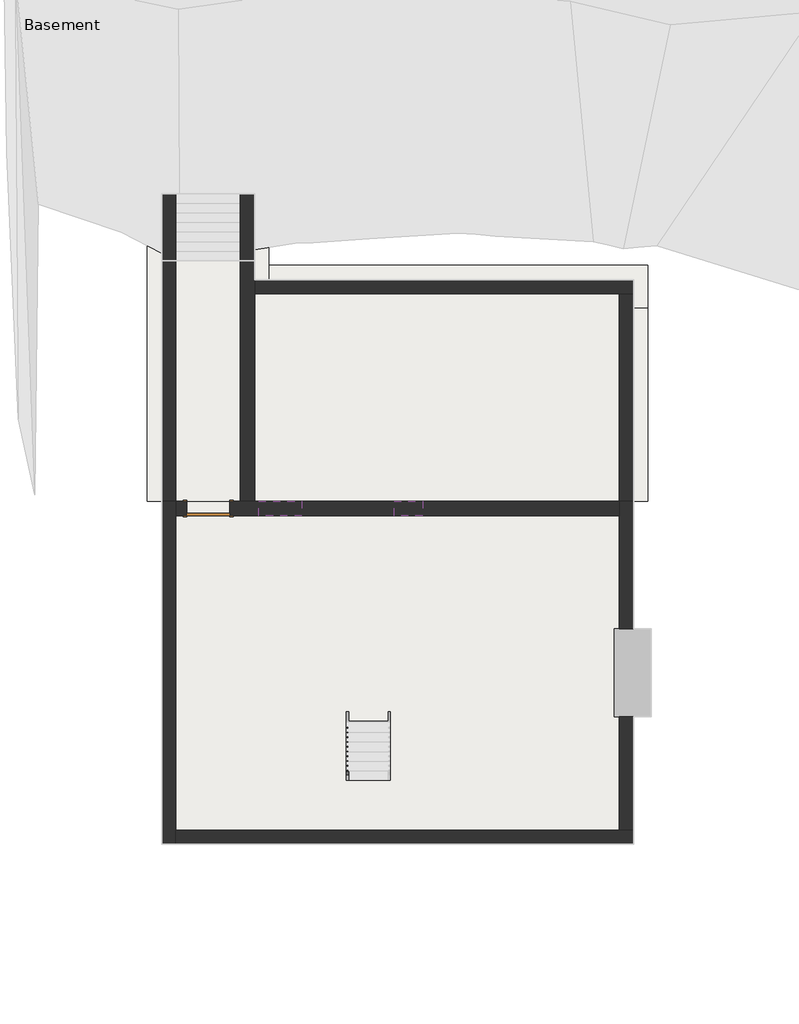
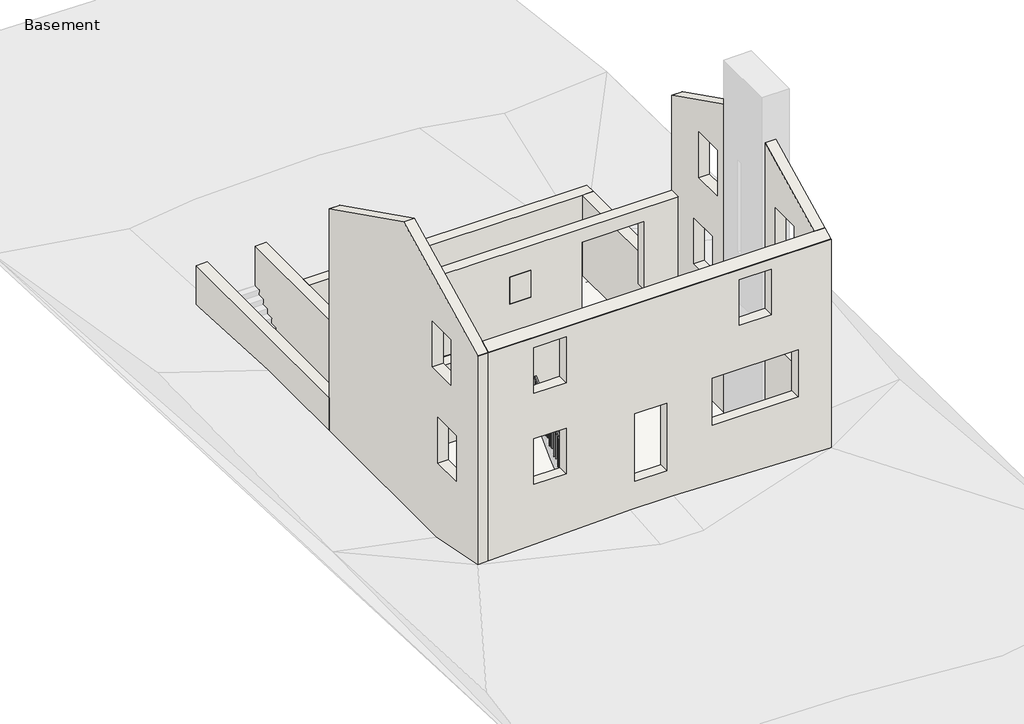
# One storey, part 1 of 2: 11 walls, 4 footings, 4 slabs, 1 door, 1 railing.
"""IFC4 building model written with IfcOpenShell, lengths in millimetres."""

import ifcopenshell
import ifcopenshell.guid

model = None  # the IFC model being written
_history = None  # IfcOwnerHistory: only IFC2X3 demands one
_inside = {}  # id of a spatial element -> (the spatial element, [elements in it])
_under = {}  # id of a project, library or spatial element -> (it, [spatial elements below it])
_declared = {}  # id of a project -> (the project, [libraries it declares])
_typed = {}  # id of a type object -> (the type object, [elements of that type])
_made_of = {}  # id of a material, layer set ... -> (it, [elements and type objects made of it])


def new_model(schema):
    """Start an empty IFC model of exactly this schema.

    Asked for "IFC4X3", IfcOpenShell would pick the latest addendum, in which some entities
    have other attributes; the version numbers below select the first issue.
    IFC2X3 requires an IfcOwnerHistory on every rooted entity: one is made here for all.
    """
    global model, _history
    if schema == "IFC4X3":
        model = ifcopenshell.file(schema_version=(4, 3, 0, 0))
    else:
        model = ifcopenshell.file(schema=schema)
    _inside.clear()
    _under.clear()
    _declared.clear()
    _typed.clear()
    _made_of.clear()
    _history = None
    if model.schema == "IFC2X3":
        org = make("IfcOrganization", Name="unknown")
        user = make(
            "IfcPersonAndOrganization",
            ThePerson=make("IfcPerson", FamilyName="unknown"),
            TheOrganization=org,
        )
        app = make(
            "IfcApplication",
            ApplicationDeveloper=org,
            Version="unknown",
            ApplicationFullName="unknown",
            ApplicationIdentifier="unknown",
        )
        _history = make(
            "IfcOwnerHistory",
            OwningUser=user,
            OwningApplication=app,
            ChangeAction="ADDED",
            CreationDate=0,
        )
    return model


def make(cls, **values):
    """One entity of the class cls with the attributes given. An attribute that is None is left unset."""
    return model.create_entity(
        cls, **{name: value for name, value in values.items() if value is not None}
    )


def rooted(cls, **values):
    """An entity with a GlobalId (a new one), such as an element, a storey or a relation."""
    return make(cls, GlobalId=ifcopenshell.guid.new(), OwnerHistory=_history, **values)


def si_unit(unit_type, name, prefix=None):
    """IfcSIUnit, for example si_unit("LENGTHUNIT", "METRE", prefix="MILLI")."""
    return make("IfcSIUnit", UnitType=unit_type, Prefix=prefix, Name=name)


def assignment(units):
    """IfcUnitAssignment: the units of a project."""
    return None if units is None else make("IfcUnitAssignment", Units=units)


def point(xyz):
    """IfcCartesianPoint."""
    return None if xyz is None else make("IfcCartesianPoint", Coordinates=xyz)


def direction(xyz):
    """IfcDirection."""
    return None if xyz is None else make("IfcDirection", DirectionRatios=xyz)


def frame(location, z_axis=None, x_axis=None):
    """IfcAxis2Placement3D, a coordinate frame: its origin and axes. An axis left out is left unset."""
    return make(
        "IfcAxis2Placement3D",
        Location=point(location),
        Axis=direction(z_axis),
        RefDirection=direction(x_axis),
    )


def origin():
    """The frame at (0, 0, 0) with its axes left unset."""
    return frame((0.0, 0.0, 0.0))


def origin_with_axes():
    """The frame at (0, 0, 0) with the z axis (0, 0, 1) and the x axis (1, 0, 0) written out."""
    return frame((0.0, 0.0, 0.0), z_axis=(0.0, 0.0, 1.0), x_axis=(1.0, 0.0, 0.0))


def place(relative_to, where):
    """IfcLocalPlacement: puts the frame where relative to a parent placement (None: the world)."""
    return make(
        "IfcLocalPlacement", PlacementRelTo=relative_to, RelativePlacement=where
    )


def context(
    kind, dimensions, precision=None, world=None, true_north=None, identifier=None
):
    """IfcGeometricRepresentationContext, for example the 3D "Model" context."""
    return make(
        "IfcGeometricRepresentationContext",
        ContextIdentifier=identifier,
        ContextType=kind,
        CoordinateSpaceDimension=dimensions,
        Precision=precision,
        WorldCoordinateSystem=world,
        TrueNorth=true_north,
    )


def project(units=None, contexts=None):
    """IfcProject with its units and contexts."""
    return rooted(
        "IfcProject",
        Name="project",
        RepresentationContexts=contexts,
        UnitsInContext=assignment(units),
    )


def spatial(cls, under=None, at=None, **own):
    """A site, building, storey or space (cls), placed at a placement, below another one or the project."""
    s = rooted(cls, ObjectPlacement=at, **own)
    if under is not None:
        _under.setdefault(under.id(), (under, []))[1].append(s)
    return s


def polyline(points):
    """IfcPolyline through the points."""
    return make("IfcPolyline", Points=[point(p) for p in points])


def outline(outer, holes=None, kind="AREA"):
    """IfcArbitraryClosedProfileDef: a profile drawn as a closed curve; with holes, ...WithVoids."""
    if holes is None:
        return make("IfcArbitraryClosedProfileDef", ProfileType=kind, OuterCurve=outer)
    return make(
        "IfcArbitraryProfileDefWithVoids",
        ProfileType=kind,
        OuterCurve=outer,
        InnerCurves=holes,
    )


def extrude(swept, where, along, depth):
    """IfcExtrudedAreaSolid: the profile swept, set in the frame where, extruded along a direction by depth."""
    return make(
        "IfcExtrudedAreaSolid",
        SweptArea=swept,
        Position=where,
        ExtrudedDirection=direction(along),
        Depth=depth,
    )


def faces_of(points, faces, orient=None, outer=None):
    """IfcFace entities. A face is a list of loops; a loop is a list of indices into points, from 0.

    orient and outer hold one flag for each loop. By default every Orientation is true, the
    first loop of a face is its IfcFaceOuterBound and the others are IfcFaceBound.
    """
    made = []
    for i, loops in enumerate(faces):
        bounds = []
        for j, loop in enumerate(loops):
            is_outer = j == 0 if outer is None else outer[i][j]
            bounds.append(
                make(
                    "IfcFaceOuterBound" if is_outer else "IfcFaceBound",
                    Bound=make("IfcPolyLoop", Polygon=[points[k] for k in loop]),
                    Orientation=True if orient is None else orient[i][j],
                )
            )
        made.append(make("IfcFace", Bounds=bounds))
    return made


def faceted_brep(points, faces, orient=None, outer=None, voids=None):
    """IfcFacetedBrep: a solid bounded by flat faces; with voids (closed shells), ...WithVoids."""
    shared = [point(p) for p in points]
    hull = make("IfcClosedShell", CfsFaces=faces_of(shared, faces, orient, outer))
    if voids is None:
        return make("IfcFacetedBrep", Outer=hull)
    return make(
        "IfcFacetedBrepWithVoids",
        Outer=hull,
        Voids=[
            make(cls, CfsFaces=faces_of(shared, fs, o, b)) for cls, fs, o, b in voids
        ],
    )


def shape(context_of_items, identifier, shape_type, items):
    """IfcShapeRepresentation: the items that make up one representation, for example the "Body"."""
    return make(
        "IfcShapeRepresentation",
        ContextOfItems=context_of_items,
        RepresentationIdentifier=identifier,
        RepresentationType=shape_type,
        Items=items,
    )


def source(mapping_origin, context_of_items, identifier, shape_type, items):
    """IfcRepresentationMap: a shape defined once, which mapped items show again and again."""
    return make(
        "IfcRepresentationMap",
        MappingOrigin=mapping_origin,
        MappedRepresentation=shape(context_of_items, identifier, shape_type, items),
    )


def transform(
    local_origin,
    x_axis=None,
    y_axis=None,
    z_axis=None,
    scale=None,
    scale2=None,
    scale3=None,
    uniform=True,
):
    """IfcCartesianTransformationOperator3D, or its non-uniform kind. x_axis, y_axis, z_axis: its Axis1, 2, 3."""
    if uniform:
        return make(
            "IfcCartesianTransformationOperator3D",
            Axis1=direction(x_axis),
            Axis2=direction(y_axis),
            LocalOrigin=point(local_origin),
            Scale=scale,
            Axis3=direction(z_axis),
        )
    return make(
        "IfcCartesianTransformationOperator3DnonUniform",
        Axis1=direction(x_axis),
        Axis2=direction(y_axis),
        LocalOrigin=point(local_origin),
        Scale=scale,
        Axis3=direction(z_axis),
        Scale2=scale2,
        Scale3=scale3,
    )


def mapped(mapping_source, mapping_target):
    """IfcMappedItem: shows the shape of a source again, moved by a transform."""
    return make(
        "IfcMappedItem", MappingSource=mapping_source, MappingTarget=mapping_target
    )


def made_of(thing, what):
    """Note that an element or type object is made of a material, layer set ...; save() writes the relation."""
    if what is not None:
        _made_of.setdefault(what.id(), (what, []))[1].append(thing)
    return thing


def element(
    cls,
    number,
    at=None,
    inside=None,
    cuts=None,
    type_object=None,
    material=None,
    context=None,
    identifier="Body",
    shape_type=None,
    held_by="IfcProductDefinitionShape",
    body=None,
    shapes=None,
    **own,
):
    """One element of the class cls, such as IfcWall. Its Tag is "e" and its number.

    at: its placement. inside: the storey or other place that contains it. cuts: it is an
    opening in that element (IfcRelVoidsElement). A single representation is given by context,
    identifier, shape_type and body (its items); several are given by shapes. held_by: the class
    of the entity that holds the representations. save() writes the other relations.
    """
    e = rooted(cls, Tag="e%d" % number, ObjectPlacement=at, **own)
    if body is not None:
        shapes = [shape(context, identifier, shape_type, body)]
    if shapes is not None:
        e.Representation = make(held_by, Representations=shapes)
    if inside is not None:
        _inside.setdefault(inside.id(), (inside, []))[1].append(e)
    if cuts is not None:
        rooted(
            "IfcRelVoidsElement", RelatingBuildingElement=cuts, RelatedOpeningElement=e
        )
    if type_object is not None:
        _typed.setdefault(type_object.id(), (type_object, []))[1].append(e)
    return made_of(e, material)


def aggregate(whole, parts):
    """IfcRelAggregates: a whole, such as a stair, and the parts it consists of."""
    return rooted("IfcRelAggregates", RelatingObject=whole, RelatedObjects=parts)


def save(model, path):
    """Write the relations noted so far, then the file.

    IfcRelAggregates (storeys below a building ...), IfcRelContainedInSpatialStructure (elements
    in a storey), IfcRelDefinesByType, IfcRelAssociatesMaterial and IfcRelDeclares: one each for
    every whole, place, type object, material and project.
    """
    for whole, parts in _under.values():
        aggregate(whole, parts)
    for where, things in _inside.values():
        rooted(
            "IfcRelContainedInSpatialStructure",
            RelatedElements=things,
            RelatingStructure=where,
        )
    for kind, things in _typed.values():
        rooted("IfcRelDefinesByType", RelatedObjects=things, RelatingType=kind)
    for what, things in _made_of.values():
        rooted("IfcRelAssociatesMaterial", RelatedObjects=things, RelatingMaterial=what)
    for by, libraries in _declared.values():
        rooted("IfcRelDeclares", RelatingContext=by, RelatedDefinitions=libraries)
    model.write(path)


def door_03272193(model_context):
    return source(origin(), model_context, "Body", "SweptSolid", [
        extrude(outline(polyline([(2209.8, -533.4), (0.0, -533.4), (0.0, -457.2), (2133.6, -457.2), (2133.6, 457.2), (0.0, 457.2), (0.0, 533.4), (2209.8, 533.4), (2209.8, -533.4)])), frame((0.0, 152.4, 0.0), z_axis=(0.0, 1.0, 0.0), x_axis=(0.0, 0.0, 1.0)), (0.0, 0.0, 1.0), 25.4),
        extrude(outline(polyline([(2209.8, 533.4), (2209.8, -533.4), (0.0, -533.4), (0.0, -457.2), (2133.6, -457.2), (2133.6, 457.2), (0.0, 457.2), (0.0, 533.4), (2209.8, 533.4)])), frame((0.0, -177.8, 0.0), z_axis=(0.0, 1.0, 0.0), x_axis=(0.0, 0.0, 1.0)), (0.0, 0.0, 1.0), 25.4),
        extrude(outline(polyline([(457.2, 101.6), (-457.2, 101.6), (-457.2, 152.4), (457.2, 152.4), (457.2, 101.6)])), origin_with_axes(), (0.0, 0.0, 1.0), 2133.6),
    ])


model = new_model("IFC4")

# Units and contexts
model_context = context("Model", 3, world=origin())
ifc_project = project(units=[si_unit("LENGTHUNIT", "METRE", prefix="MILLI")], contexts=[model_context])

# Site, building, storey
site = spatial("IfcSite", under=ifc_project)
building = spatial("IfcBuilding", under=site)
storey = spatial("IfcBuildingStorey", under=building, Name="Basement", Elevation=-2667.0)

# Door
placement = place(None, origin())
door_shape = door_03272193(model_context)
element("IfcDoor", 1, ObjectType="Single-Flush : 36\" x 84\"", at=placement, inside=storey, context=model_context, shape_type="MappedRepresentation", body=[
    mapped(door_shape, transform((-4998.5803068, 2999.6888758, -2667.0), x_axis=(-1.0, 0.0, 0.0), y_axis=(0.0, -1.0, 0.0), z_axis=(0.0, 0.0, 1.0))),
])

# Footings
element("IfcFooting", 2, ObjectType="Bearing Footing - 36\" x 12\"", at=placement, inside=storey, context=model_context, shape_type="SweptSolid", body=[
    extrude(outline(polyline([(-5379.5803068, 3152.0888758), (-6293.9803068, 3152.0888758), (-6293.9803068, 10010.0888758), (-5379.5803068, 10010.0888758), (-5379.5803068, 3152.0888758)])), frame((0.0, 0.0, -3073.4), z_axis=(0.0, 0.0, 1.0), x_axis=(1.0, 0.0, 0.0)), (0.0, 0.0, 1.0), 304.8),
])
element("IfcFooting", 3, ObjectType="Bearing Footing - 36\" x 12\"", at=placement, inside=storey, context=model_context, shape_type="Brep", body=[
    faceted_brep([(-3703.1803068, 7266.8888758, -2768.6), (3459.6196932, 7266.8888758, -2768.6), (4374.0196932, 7266.8888758, -2768.6), (4374.0196932, 8181.2888758, -2768.6), (-3703.1803068, 8181.2888758, -2768.6), (-3703.1803068, 8181.2888758, -3073.4), (4374.0196932, 8181.2888758, -3073.4), (-3703.1803068, 7266.8888758, -3073.4), (4374.0196932, 7266.8888758, -3073.4), (3459.6196932, 7266.8888758, -3073.4)], [[[0, 1, 2, 3, 4]], [[5, 4, 3, 6]], [[7, 5, 6, 8, 9]], [[0, 7, 9, 8, 2, 1]], [[0, 4, 5, 7]], [[3, 2, 8, 6]]]),
])
element("IfcFooting", 4, ObjectType="Bearing Footing - 36\" x 12\"", at=placement, inside=storey, context=model_context, shape_type="SweptSolid", body=[
    extrude(outline(polyline([(4374.0196932, 3152.0888758), (3459.6196932, 3152.0888758), (3459.6196932, 7266.8888758), (4374.0196932, 7266.8888758), (4374.0196932, 3152.0888758)])), frame((0.0, 0.0, -3073.4), z_axis=(0.0, 0.0, 1.0), x_axis=(1.0, 0.0, 0.0)), (0.0, 0.0, 1.0), 304.8),
])
element("IfcFooting", 5, ObjectType="Bearing Footing - 36\" x 12\"", at=placement, inside=storey, context=model_context, shape_type="Brep", body=[
    faceted_brep([(-3703.1803068, 3152.0888758, -2768.6), (-4617.5803068, 3152.0888758, -2768.6), (-4617.5803068, 3152.0888758, -3073.4), (-3703.1803068, 3152.0888758, -3073.4), (-4617.5803068, 10010.0888758, -2768.6), (-3703.1803068, 10010.0888758, -2768.6), (-3703.1803068, 10010.0888758, -3073.4), (-4617.5803068, 10010.0888758, -3073.4), (-3703.1803068, 7266.8888758, -2768.6), (-3703.1803068, 8181.2888758, -2768.6), (-3703.1803068, 8181.2888758, -3073.4), (-3703.1803068, 7266.8888758, -3073.4)], [[[0, 1, 2, 3]], [[4, 5, 6, 7]], [[0, 8, 9, 5, 4, 1]], [[2, 1, 4, 7]], [[3, 2, 7, 6, 10, 11]], [[0, 3, 11, 10, 6, 5, 9, 8]]]),
])

# Railing
element("IfcRailing", 6, ObjectType="Handrail - Rectangular", at=placement, inside=storey, context=model_context, shape_type="SweptSolid", body=[
    extrude(outline(polyline([(-2791.5111242, -1631.7331862), (-2791.5111242, -1562.1), (-149.9111242, 914.4), (-149.9111242, 844.7668138), (-2791.5111242, -1631.7331862)])), frame((-2052.1803068, 0.0, 0.0), z_axis=(1.0, 0.0, 0.0), x_axis=(0.0, 1.0, 0.0)), (0.0, 0.0, 1.0), 50.8),
    extrude(outline(polyline([(-241.9861242, 758.4465013), (-241.9861242, -190.5), (-261.0361242, -190.5), (-261.0361242, 740.5871263), (-241.9861242, 758.4465013)])), frame((-2036.3053068, 0.0, 0.0), z_axis=(1.0, 0.0, 0.0), x_axis=(0.0, 1.0, 0.0)), (0.0, 0.0, 1.0), 19.05),
    extrude(outline(polyline([(-343.5861242, 663.1965013), (-343.5861242, -190.5), (-362.6361242, -190.5), (-362.6361242, 645.3371263), (-343.5861242, 663.1965013)])), frame((-2036.3053068, 0.0, 0.0), z_axis=(1.0, 0.0, 0.0), x_axis=(0.0, 1.0, 0.0)), (0.0, 0.0, 1.0), 19.05),
    extrude(outline(polyline([(-445.1861242, 567.9465013), (-445.1861242, -381.0), (-464.2361242, -381.0), (-464.2361242, 550.0871263), (-445.1861242, 567.9465013)])), frame((-2036.3053068, 0.0, 0.0), z_axis=(1.0, 0.0, 0.0), x_axis=(0.0, 1.0, 0.0)), (0.0, 0.0, 1.0), 19.05),
    extrude(outline(polyline([(-546.7861242, 472.6965013), (-546.7861242, -381.0), (-565.8361242, -381.0), (-565.8361242, 454.8371263), (-546.7861242, 472.6965013)])), frame((-2036.3053068, 0.0, 0.0), z_axis=(1.0, 0.0, 0.0), x_axis=(0.0, 1.0, 0.0)), (0.0, 0.0, 1.0), 19.05),
    extrude(outline(polyline([(-648.3861242, 377.4465013), (-648.3861242, -571.5), (-667.4361242, -571.5), (-667.4361242, 359.5871263), (-648.3861242, 377.4465013)])), frame((-2036.3053068, 0.0, 0.0), z_axis=(1.0, 0.0, 0.0), x_axis=(0.0, 1.0, 0.0)), (0.0, 0.0, 1.0), 19.05),
    extrude(outline(polyline([(-749.9861242, 282.1965013), (-749.9861242, -571.5), (-769.0361242, -571.5), (-769.0361242, 264.3371263), (-749.9861242, 282.1965013)])), frame((-2036.3053068, 0.0, 0.0), z_axis=(1.0, 0.0, 0.0), x_axis=(0.0, 1.0, 0.0)), (0.0, 0.0, 1.0), 19.05),
    extrude(outline(polyline([(-851.5861242, 186.9465013), (-851.5861242, -762.0), (-870.6361242, -762.0), (-870.6361242, 169.0871263), (-851.5861242, 186.9465013)])), frame((-2036.3053068, 0.0, 0.0), z_axis=(1.0, 0.0, 0.0), x_axis=(0.0, 1.0, 0.0)), (0.0, 0.0, 1.0), 19.05),
    extrude(outline(polyline([(-953.1861242, 91.6965013), (-953.1861242, -762.0), (-972.2361242, -762.0), (-972.2361242, 73.8371263), (-953.1861242, 91.6965013)])), frame((-2036.3053068, 0.0, 0.0), z_axis=(1.0, 0.0, 0.0), x_axis=(0.0, 1.0, 0.0)), (0.0, 0.0, 1.0), 19.05),
    extrude(outline(polyline([(-1054.7861242, -3.5534987), (-1054.7861242, -952.5), (-1073.8361242, -952.5), (-1073.8361242, -21.4128737), (-1054.7861242, -3.5534987)])), frame((-2036.3053068, 0.0, 0.0), z_axis=(1.0, 0.0, 0.0), x_axis=(0.0, 1.0, 0.0)), (0.0, 0.0, 1.0), 19.05),
    extrude(outline(polyline([(-1156.3861242, -98.8034987), (-1156.3861242, -952.5), (-1175.4361242, -952.5), (-1175.4361242, -116.6628737), (-1156.3861242, -98.8034987)])), frame((-2036.3053068, 0.0, 0.0), z_axis=(1.0, 0.0, 0.0), x_axis=(0.0, 1.0, 0.0)), (0.0, 0.0, 1.0), 19.05),
    extrude(outline(polyline([(-1257.9861242, -194.0534987), (-1257.9861242, -1143.0), (-1277.0361242, -1143.0), (-1277.0361242, -211.9128737), (-1257.9861242, -194.0534987)])), frame((-2036.3053068, 0.0, 0.0), z_axis=(1.0, 0.0, 0.0), x_axis=(0.0, 1.0, 0.0)), (0.0, 0.0, 1.0), 19.05),
    extrude(outline(polyline([(-1359.5861242, -289.3034987), (-1359.5861242, -1143.0), (-1378.6361242, -1143.0), (-1378.6361242, -307.1628737), (-1359.5861242, -289.3034987)])), frame((-2036.3053068, 0.0, 0.0), z_axis=(1.0, 0.0, 0.0), x_axis=(0.0, 1.0, 0.0)), (0.0, 0.0, 1.0), 19.05),
    extrude(outline(polyline([(-1461.1861242, -384.5534987), (-1461.1861242, -1333.5), (-1480.2361242, -1333.5), (-1480.2361242, -402.4128737), (-1461.1861242, -384.5534987)])), frame((-2036.3053068, 0.0, 0.0), z_axis=(1.0, 0.0, 0.0), x_axis=(0.0, 1.0, 0.0)), (0.0, 0.0, 1.0), 19.05),
    extrude(outline(polyline([(-1562.7861242, -479.8034987), (-1562.7861242, -1333.5), (-1581.8361242, -1333.5), (-1581.8361242, -497.6628737), (-1562.7861242, -479.8034987)])), frame((-2036.3053068, 0.0, 0.0), z_axis=(1.0, 0.0, 0.0), x_axis=(0.0, 1.0, 0.0)), (0.0, 0.0, 1.0), 19.05),
    extrude(outline(polyline([(-1664.3861242, -575.0534987), (-1664.3861242, -1524.0), (-1683.4361242, -1524.0), (-1683.4361242, -592.9128737), (-1664.3861242, -575.0534987)])), frame((-2036.3053068, 0.0, 0.0), z_axis=(1.0, 0.0, 0.0), x_axis=(0.0, 1.0, 0.0)), (0.0, 0.0, 1.0), 19.05),
    extrude(outline(polyline([(-1765.9861242, -670.3034987), (-1765.9861242, -1524.0), (-1785.0361242, -1524.0), (-1785.0361242, -688.1628737), (-1765.9861242, -670.3034987)])), frame((-2036.3053068, 0.0, 0.0), z_axis=(1.0, 0.0, 0.0), x_axis=(0.0, 1.0, 0.0)), (0.0, 0.0, 1.0), 19.05),
    extrude(outline(polyline([(-1867.5861242, -765.5534987), (-1867.5861242, -1714.5), (-1886.6361242, -1714.5), (-1886.6361242, -783.4128737), (-1867.5861242, -765.5534987)])), frame((-2036.3053068, 0.0, 0.0), z_axis=(1.0, 0.0, 0.0), x_axis=(0.0, 1.0, 0.0)), (0.0, 0.0, 1.0), 19.05),
    extrude(outline(polyline([(-1969.1861242, -860.8034987), (-1969.1861242, -1714.5), (-1988.2361242, -1714.5), (-1988.2361242, -878.6628737), (-1969.1861242, -860.8034987)])), frame((-2036.3053068, 0.0, 0.0), z_axis=(1.0, 0.0, 0.0), x_axis=(0.0, 1.0, 0.0)), (0.0, 0.0, 1.0), 19.05),
    extrude(outline(polyline([(-2070.7861242, -956.0534987), (-2070.7861242, -1905.0), (-2089.8361242, -1905.0), (-2089.8361242, -973.9128737), (-2070.7861242, -956.0534987)])), frame((-2036.3053068, 0.0, 0.0), z_axis=(1.0, 0.0, 0.0), x_axis=(0.0, 1.0, 0.0)), (0.0, 0.0, 1.0), 19.05),
    extrude(outline(polyline([(-2172.3861242, -1051.3034987), (-2172.3861242, -1905.0), (-2191.4361242, -1905.0), (-2191.4361242, -1069.1628737), (-2172.3861242, -1051.3034987)])), frame((-2036.3053068, 0.0, 0.0), z_axis=(1.0, 0.0, 0.0), x_axis=(0.0, 1.0, 0.0)), (0.0, 0.0, 1.0), 19.05),
    extrude(outline(polyline([(-2273.9861242, -1146.5534987), (-2273.9861242, -2095.5), (-2293.0361242, -2095.5), (-2293.0361242, -1164.4128737), (-2273.9861242, -1146.5534987)])), frame((-2036.3053068, 0.0, 0.0), z_axis=(1.0, 0.0, 0.0), x_axis=(0.0, 1.0, 0.0)), (0.0, 0.0, 1.0), 19.05),
    extrude(outline(polyline([(-2375.5861242, -1241.8034987), (-2375.5861242, -2095.5), (-2394.6361242, -2095.5), (-2394.6361242, -1259.6628737), (-2375.5861242, -1241.8034987)])), frame((-2036.3053068, 0.0, 0.0), z_axis=(1.0, 0.0, 0.0), x_axis=(0.0, 1.0, 0.0)), (0.0, 0.0, 1.0), 19.05),
    extrude(outline(polyline([(-2477.1861242, -1337.0534987), (-2477.1861242, -2286.0), (-2496.2361242, -2286.0), (-2496.2361242, -1354.9128737), (-2477.1861242, -1337.0534987)])), frame((-2036.3053068, 0.0, 0.0), z_axis=(1.0, 0.0, 0.0), x_axis=(0.0, 1.0, 0.0)), (0.0, 0.0, 1.0), 19.05),
    extrude(outline(polyline([(-2578.7861242, -1432.3034987), (-2578.7861242, -2286.0), (-2597.8361242, -2286.0), (-2597.8361242, -1450.1628737), (-2578.7861242, -1432.3034987)])), frame((-2036.3053068, 0.0, 0.0), z_axis=(1.0, 0.0, 0.0), x_axis=(0.0, 1.0, 0.0)), (0.0, 0.0, 1.0), 19.05),
    extrude(outline(polyline([(-2680.3861242, -1527.5534987), (-2680.3861242, -2476.5), (-2699.4361242, -2476.5), (-2699.4361242, -1545.4128737), (-2680.3861242, -1527.5534987)])), frame((-2036.3053068, 0.0, 0.0), z_axis=(1.0, 0.0, 0.0), x_axis=(0.0, 1.0, 0.0)), (0.0, 0.0, 1.0), 19.05),
    extrude(outline(polyline([(-149.9111242, 844.7668138), (-149.9111242, -190.5), (-168.9611242, -190.5), (-168.9611242, 826.9074388), (-149.9111242, 844.7668138)])), frame((-2036.3053068, 0.0, 0.0), z_axis=(1.0, 0.0, 0.0), x_axis=(0.0, 1.0, 0.0)), (0.0, 0.0, 1.0), 19.05),
    extrude(outline(polyline([(-2772.4611242, -1613.8738112), (-2772.4611242, -2476.5), (-2791.5111242, -2476.5), (-2791.5111242, -1631.7331862), (-2772.4611242, -1613.8738112)])), frame((-2036.3053068, 0.0, 0.0), z_axis=(1.0, 0.0, 0.0), x_axis=(0.0, 1.0, 0.0)), (0.0, 0.0, 1.0), 19.05),
])

# Slabs
element("IfcSlab", 7, ObjectType="4\" Concrete", at=placement, inside=storey, context=model_context, shape_type="SweptSolid", body=[
    extrude(outline(polyline([(-5684.3803068, 8384.4888758), (-4312.7803068, 8384.4888758), (-4312.7803068, 3152.0888758), (-5684.3803068, 3152.0888758), (-5684.3803068, 8384.4888758)])), frame((0.0, 0.0, -2768.6), z_axis=(0.0, 0.0, 1.0), x_axis=(1.0, 0.0, 0.0)), (0.0, 0.0, 1.0), 101.6),
])
element("IfcSlab", 8, ObjectType="Pad 1", at=placement, inside=storey, context=model_context, shape_type="SweptSolid", body=[
    extrude(outline(polyline([(4069.2196932, 434.2888758), (4450.2196932, 434.2888758), (4450.2196932, -1445.3111242), (4069.2196932, -1445.3111242), (4069.2196932, -4163.1111242), (-5989.1803068, -4163.1111242), (-5989.1803068, 3152.0888758), (4069.2196932, 3152.0888758), (4069.2196932, 434.2888758)])), frame((0.0, 0.0, -3073.4), z_axis=(0.0, 0.0, 1.0), x_axis=(1.0, 0.0, 0.0)), (0.0, 0.0, 1.0), 304.8),
])
element("IfcSlab", 9, ObjectType="Pad 1", at=placement, inside=storey, context=model_context, shape_type="SweptSolid", body=[
    extrude(outline(polyline([(-5989.1803068, 8275.4102719), (-4007.9803068, 8275.4102719), (-4007.9803068, 7876.4888758), (4069.2196932, 7876.4888758), (4069.2196932, 3152.0888758), (-5989.1803068, 3152.0888758), (-5989.1803068, 8275.4102719)])), frame((0.0, 0.0, -3073.4), z_axis=(0.0, 0.0, 1.0), x_axis=(1.0, 0.0, 0.0)), (0.0, 0.0, 1.0), 304.8),
])
element("IfcSlab", 10, ObjectType="Under Stairs", at=placement, inside=storey, context=model_context, shape_type="SweptSolid", body=[
    extrude(outline(polyline([(9705.2888758, -1653.200634), (8275.4102719, -2776.6756068), (8275.4102719, -2768.6), (9705.2888758, -1645.1250272), (9705.2888758, -1653.200634)])), frame((-5989.1803068, 0.0, 0.0), z_axis=(1.0, 0.0, 0.0), x_axis=(0.0, 1.0, 0.0)), (0.0, 0.0, 1.0), 1981.2),
])

# Walls
element("IfcWall", 11, ObjectType="Foundation - 12\" Concrete", at=placement, inside=storey, context=model_context, shape_type="Brep", body=[
    faceted_brep([(-5684.3803068, 3152.0888758, -2768.6), (-5684.3803068, 8384.4888758, -2768.6), (-5684.3803068, 9705.2888758, -2768.6), (-5684.3803068, 9705.2888758, -349.25), (-5684.3803068, 3152.0888758, -349.25), (-5684.3803068, 3152.0888758, -2667.0), (-5989.1803068, 3152.0888758, -2768.6), (-5989.1803068, 3152.0888758, -349.25), (-5989.1803068, 9705.2888758, -349.25), (-5989.1803068, 9705.2888758, -2768.6)], [[[0, 1, 2, 3, 4, 5]], [[6, 7, 8, 9]], [[2, 1, 0, 6, 9]], [[3, 2, 9, 8]], [[4, 3, 8, 7]], [[0, 5, 4, 7, 6]]]),
])
element("IfcWall", 12, ObjectType="Foundation - 12\" Concrete", at=placement, inside=storey, context=model_context, shape_type="Brep", body=[
    faceted_brep([(-4007.9803068, 7571.6888758, -2768.6), (3764.4196932, 7571.6888758, -2768.6), (4069.2196932, 7571.6888758, -2768.6), (4069.2196932, 7571.6888758, -349.25), (3764.4196932, 7571.6888758, -349.25), (-4007.9803068, 7571.6888758, -349.25), (-4007.9803068, 7876.4888758, -2768.6), (-4007.9803068, 7876.4888758, -349.25), (4069.2196932, 7876.4888758, -349.25), (4069.2196932, 7876.4888758, -2768.6)], [[[0, 1, 2, 3, 4, 5]], [[6, 7, 8, 9]], [[2, 1, 0, 6, 9]], [[5, 4, 3, 8, 7]], [[3, 2, 9, 8]], [[0, 5, 7, 6]]]),
])
element("IfcWall", 13, ObjectType="Foundation - 12\" Concrete", at=placement, inside=storey, context=model_context, shape_type="Brep", body=[
    faceted_brep([(3764.4196932, 7571.6888758, -2768.6), (3764.4196932, 3152.0888758, -2768.6), (3764.4196932, 3152.0888758, -349.25), (3764.4196932, 7571.6888758, -349.25), (4069.2196932, 7571.6888758, -2768.6), (4069.2196932, 7571.6888758, -349.25), (4069.2196932, 7524.0638758, -349.25), (4069.2196932, 3152.0888758, -349.25), (4069.2196932, 3152.0888758, -2768.6)], [[[0, 1, 2, 3]], [[4, 5, 6, 7, 8]], [[1, 0, 4, 8]], [[3, 2, 7, 6, 5]], [[2, 1, 8, 7]], [[0, 3, 5, 4]]]),
])
element("IfcWall", 14, ObjectType="Foundation - 12\" Concrete", at=placement, inside=storey, context=model_context, shape_type="Brep", body=[
    faceted_brep([(-4007.9803068, 3152.0888758, -2768.6), (-4007.9803068, 7571.6888758, -2768.6), (-4007.9803068, 7876.4888758, -2768.6), (-4007.9803068, 9705.2888758, -2768.6), (-4007.9803068, 9705.2888758, -349.25), (-4007.9803068, 7876.4888758, -349.25), (-4007.9803068, 7571.6888758, -349.25), (-4007.9803068, 3152.0888758, -349.25), (-4312.7803068, 3152.0888758, -2768.6), (-4312.7803068, 3152.0888758, -2667.0), (-4312.7803068, 3152.0888758, -349.25), (-4312.7803068, 9705.2888758, -349.25), (-4312.7803068, 9705.2888758, -2768.6), (-4312.7803068, 8384.4888758, -2768.6)], [[[0, 1, 2, 3, 4, 5, 6, 7]], [[8, 9, 10, 11, 12, 13]], [[3, 2, 1, 0, 8, 13, 12]], [[4, 3, 12, 11]], [[7, 6, 5, 4, 11, 10]], [[0, 7, 10, 9, 8]]]),
])
element("IfcWall", 15, ObjectType="Generic - 12\"", at=placement, inside=storey, context=model_context, shape_type="Brep", body=[
    faceted_brep([(1021.2196932, 2847.2888758, 0.0), (1021.2196932, 2847.2888758, 2057.4), (2799.2196932, 2847.2888758, 2057.4), (2799.2196932, 2847.2888758, 0.0), (3764.4196932, 2847.2888758, 0.0), (3764.4196932, 2847.2888758, 2470.15), (-680.5803068, 2847.2888758, 2470.15), (-5684.3803068, 2847.2888758, 2470.15), (-5684.3803068, 2847.2888758, 0.0), (-5023.9803068, 2847.2888758, 0.0), (-5023.9803068, 2847.2888758, 2032.0), (-4160.3803068, 2847.2888758, 2032.0), (-4160.3803068, 2847.2888758, 0.0), (-1518.7803068, 2847.2888758, 0.0), (-1391.7803068, 2847.2888758, 0.0), (-70.9803068, 2847.2888758, 0.0), (56.0196932, 2847.2888758, 0.0), (-3919.0803068, 2847.2888758, 914.4), (-3919.0803068, 2847.2888758, 1727.2), (-3004.6803068, 2847.2888758, 1727.2), (-3004.6803068, 2847.2888758, 914.4), (-1036.1803068, 2847.2888758, 914.4), (-1036.1803068, 2847.2888758, 1727.2), (-426.5803068, 2847.2888758, 1727.2), (-426.5803068, 2847.2888758, 914.4), (1021.2196932, 3152.0888758, 2057.4), (1021.2196932, 3152.0888758, 0.0), (-4160.3803068, 3152.0888758, 0.0), (-4160.3803068, 3152.0888758, 2032.0), (-5023.9803068, 3152.0888758, 2032.0), (-5023.9803068, 3152.0888758, 0.0), (-5684.3803068, 3152.0888758, 0.0), (-5684.3803068, 3152.0888758, 2470.15), (3764.4196932, 3152.0888758, 2470.15), (3764.4196932, 3152.0888758, 0.0), (2799.2196932, 3152.0888758, 0.0), (2799.2196932, 3152.0888758, 2057.4), (-3919.0803068, 3152.0888758, 1727.2), (-3919.0803068, 3152.0888758, 914.4), (-3004.6803068, 3152.0888758, 914.4), (-3004.6803068, 3152.0888758, 1727.2), (-1036.1803068, 3152.0888758, 1727.2), (-1036.1803068, 3152.0888758, 914.4), (-426.5803068, 3152.0888758, 914.4), (-426.5803068, 3152.0888758, 1727.2)], [[[0, 1, 2, 3, 4, 5, 6, 7, 8, 9, 10, 11, 12, 13, 14, 15, 16], [17, 18, 19, 20], [21, 22, 23, 24]], [[25, 26, 27, 28, 29, 30, 31, 32, 33, 34, 35, 36], [37, 38, 39, 40], [41, 42, 43, 44]], [[25, 1, 0, 26]], [[1, 25, 36, 2]], [[2, 36, 35, 3]], [[10, 9, 30, 29]], [[11, 10, 29, 28]], [[12, 11, 28, 27]], [[9, 8, 31, 30]], [[4, 3, 35, 34]], [[0, 16, 15, 14, 13, 12, 27, 26]], [[7, 6, 5, 33, 32]], [[4, 34, 33, 5]], [[37, 18, 17, 38]], [[38, 17, 20, 39]], [[39, 20, 19, 40]], [[18, 37, 40, 19]], [[41, 22, 21, 42]], [[42, 21, 24, 43]], [[43, 24, 23, 44]], [[22, 41, 44, 23]], [[31, 8, 7, 32]]]),
    faceted_brep([(3764.4196932, 2847.2888758, -273.05), (-5684.3803068, 2847.2888758, -273.05), (-5684.3803068, 2847.2888758, -2667.0), (-5455.7803068, 2847.2888758, -2667.0), (-5455.7803068, 2847.2888758, -533.4), (-4541.3803068, 2847.2888758, -533.4), (-4541.3803068, 2847.2888758, -2667.0), (3764.4196932, 2847.2888758, -2667.0), (-5684.3803068, 3152.0888758, -273.05), (3764.4196932, 3152.0888758, -273.05), (3764.4196932, 3152.0888758, -2667.0), (-4541.3803068, 3152.0888758, -2667.0), (-4541.3803068, 3152.0888758, -533.4), (-5455.7803068, 3152.0888758, -533.4), (-5455.7803068, 3152.0888758, -2667.0), (-5684.3803068, 3152.0888758, -2667.0)], [[[0, 1, 2, 3, 4, 5, 6, 7]], [[8, 9, 10, 11, 12, 13, 14, 15]], [[10, 7, 6, 11]], [[3, 2, 15, 14]], [[1, 0, 9, 8]], [[7, 10, 9, 0]], [[13, 4, 3, 14]], [[4, 13, 12, 5]], [[5, 12, 11, 6]], [[15, 2, 1, 8]]]),
])
element("IfcWall", 16, ObjectType="Generic - 12\"", at=placement, inside=storey, context=model_context, shape_type="Brep", body=[
    faceted_brep([(-5684.3803068, -4163.1111242, -2667.0), (-5684.3803068, -3858.3111242, -2667.0), (-5684.3803068, 2847.2888758, -2667.0), (-5684.3803068, 3152.0888758, -2667.0), (-5684.3803068, 3152.0888758, -273.05), (-5684.3803068, 3152.0888758, 0.0), (-5684.3803068, 3152.0888758, 2470.15), (-5684.3803068, 2847.2888758, 2470.15), (-5684.3803068, 1450.2888758, 2470.15), (-5684.3803068, 1450.2888758, 2743.2), (-5684.3803068, 3152.0888758, 2743.2), (-5684.3803068, 3152.0888758, 5336.1342644), (-5684.3803068, 3147.820347, 5336.1342644), (-5684.3803068, -505.5111242, 7162.8), (-5684.3803068, -3858.3111242, 5486.4), (-5684.3803068, -4158.8425953, 5336.1342644), (-5684.3803068, -4163.1111242, 5336.1342644), (-5684.3803068, -3096.3111242, 914.4), (-5684.3803068, -3096.3111242, 2286.0), (-5684.3803068, -2181.9111242, 2286.0), (-5684.3803068, -2181.9111242, 914.4), (-5684.3803068, -2842.3111242, 3657.6), (-5684.3803068, -2842.3111242, 5029.2), (-5684.3803068, -1927.9111242, 5029.2), (-5684.3803068, -1927.9111242, 3657.6), (-5989.1803068, 3152.0888758, -2667.0), (-5989.1803068, -4163.1111242, -2667.0), (-5989.1803068, -4163.1111242, 5336.1342644), (-5989.1803068, -4158.8425953, 5336.1342644), (-5989.1803068, -505.5111242, 7162.8), (-5989.1803068, 3147.820347, 5336.1342644), (-5989.1803068, 3152.0888758, 5336.1342644), (-5989.1803068, -3096.3111242, 2286.0), (-5989.1803068, -3096.3111242, 914.4), (-5989.1803068, -2181.9111242, 914.4), (-5989.1803068, -2181.9111242, 2286.0), (-5989.1803068, -2842.3111242, 5029.2), (-5989.1803068, -2842.3111242, 3657.6), (-5989.1803068, -1927.9111242, 3657.6), (-5989.1803068, -1927.9111242, 5029.2), (-5801.8553068, 3152.0888758, 2743.2), (-5801.8553068, 3152.0888758, 2470.15), (-5801.8553068, 1450.2888758, 2470.15), (-5801.8553068, 1450.2888758, 2743.2)], [[[0, 1, 2, 3, 4, 5, 6, 7, 8, 9, 10, 11, 12, 13, 14, 15, 16], [17, 18, 19, 20], [21, 22, 23, 24]], [[25, 26, 27, 28, 29, 30, 31], [32, 33, 34, 35], [36, 37, 38, 39]], [[3, 2, 1, 0, 26, 25]], [[0, 16, 27, 26]], [[33, 32, 18, 17]], [[34, 33, 17, 20]], [[35, 34, 20, 19]], [[32, 35, 19, 18]], [[22, 21, 37, 36]], [[21, 24, 38, 37]], [[24, 23, 39, 38]], [[23, 22, 36, 39]], [[27, 16, 15, 28]], [[29, 28, 15, 14, 13]], [[13, 12, 30, 29]], [[12, 11, 31, 30]], [[3, 25, 31, 11, 10, 40, 41, 6, 5, 4]], [[41, 42, 8, 7, 6]], [[9, 43, 40, 10]], [[43, 42, 41, 40]], [[42, 43, 9, 8]]]),
])
element("IfcWall", 17, ObjectType="Generic - 12\"", at=placement, inside=storey, context=model_context, shape_type="Brep", body=[
    faceted_brep([(4069.2196932, -3858.3111242, -2667.0), (3764.4196932, -3858.3111242, -2667.0), (-5684.3803068, -3858.3111242, -2667.0), (-5684.3803068, -3858.3111242, 5486.4), (3764.4196932, -3858.3111242, 5486.4), (4069.2196932, -3858.3111242, 5486.4), (-1518.7803068, -3858.3111242, 0.0), (-604.3803068, -3858.3111242, 0.0), (-604.3803068, -3858.3111242, 2032.0), (-1518.7803068, -3858.3111242, 2032.0), (-3474.5803068, -3858.3111242, 914.4), (-3474.5803068, -3858.3111242, 2286.0), (-4388.9803068, -3858.3111242, 2286.0), (-4388.9803068, -3858.3111242, 914.4), (2367.4196932, -3858.3111242, 3657.6), (2367.4196932, -3858.3111242, 5029.2), (1453.0196932, -3858.3111242, 5029.2), (1453.0196932, -3858.3111242, 3657.6), (-3474.5803068, -3858.3111242, 3657.6), (-3474.5803068, -3858.3111242, 5029.2), (-4388.9803068, -3858.3111242, 5029.2), (-4388.9803068, -3858.3111242, 3657.6), (3129.4196932, -3858.3111242, 2336.8), (691.0196932, -3858.3111242, 2336.8), (691.0196932, -3858.3111242, 914.4), (3129.4196932, -3858.3111242, 914.4), (-5684.3803068, -4163.1111242, -2667.0), (4069.2196932, -4163.1111242, -2667.0), (4069.2196932, -4163.1111242, 5336.1342644), (-5684.3803068, -4163.1111242, 5336.1342644), (-604.3803068, -4163.1111242, 0.0), (-1518.7803068, -4163.1111242, 0.0), (-1518.7803068, -4163.1111242, 2032.0), (-604.3803068, -4163.1111242, 2032.0), (-3474.5803068, -4163.1111242, 2286.0), (-3474.5803068, -4163.1111242, 914.4), (-4388.9803068, -4163.1111242, 914.4), (-4388.9803068, -4163.1111242, 2286.0), (2367.4196932, -4163.1111242, 5029.2), (2367.4196932, -4163.1111242, 3657.6), (1453.0196932, -4163.1111242, 3657.6), (1453.0196932, -4163.1111242, 5029.2), (-3474.5803068, -4163.1111242, 5029.2), (-3474.5803068, -4163.1111242, 3657.6), (-4388.9803068, -4163.1111242, 3657.6), (-4388.9803068, -4163.1111242, 5029.2), (3129.4196932, -4163.1111242, 914.4), (691.0196932, -4163.1111242, 914.4), (691.0196932, -4163.1111242, 2336.8), (3129.4196932, -4163.1111242, 2336.8), (4069.2196932, -4158.8425953, 5336.1342644), (-5684.3803068, -4158.8425953, 5336.1342644)], [[[0, 1, 2, 3, 4, 5], [6, 7, 8, 9], [10, 11, 12, 13], [14, 15, 16, 17], [18, 19, 20, 21], [22, 23, 24, 25]], [[26, 27, 28, 29], [30, 31, 32, 33], [34, 35, 36, 37], [38, 39, 40, 41], [42, 43, 44, 45], [46, 47, 48, 49]], [[2, 1, 0, 27, 26]], [[0, 5, 50, 28, 27]], [[3, 2, 26, 29, 51]], [[31, 30, 7, 6]], [[32, 31, 6, 9]], [[33, 32, 9, 8]], [[30, 33, 8, 7]], [[35, 34, 11, 10]], [[36, 35, 10, 13]], [[37, 36, 13, 12]], [[34, 37, 12, 11]], [[24, 47, 46, 25]], [[48, 23, 22, 49]], [[23, 48, 47, 24]], [[25, 46, 49, 22]], [[15, 14, 39, 38]], [[14, 17, 40, 39]], [[17, 16, 41, 40]], [[16, 15, 38, 41]], [[19, 18, 43, 42]], [[18, 21, 44, 43]], [[21, 20, 45, 44]], [[20, 19, 42, 45]], [[5, 4, 3, 51, 50]], [[29, 28, 50, 51]]]),
])
element("IfcWall", 18, ObjectType="Generic - 12\"", at=placement, inside=storey, context=model_context, shape_type="Brep", body=[
    faceted_brep([(3764.4196932, 3152.0888758, -2667.0), (3764.4196932, 2847.2888758, -2667.0), (3764.4196932, 434.2888758, -2667.0), (3764.4196932, 434.2888758, 6692.9), (3764.4196932, 2847.2888758, 5486.4), (3764.4196932, 3147.820347, 5336.1342644), (3764.4196932, 3152.0888758, 5336.1342644), (3764.4196932, 3152.0888758, 2743.2), (3764.4196932, 3152.0888758, 2470.15), (3764.4196932, 3152.0888758, 0.0), (3764.4196932, 3152.0888758, -273.05), (3764.4196932, 2085.2888758, 2286.0), (3764.4196932, 1170.8888758, 2286.0), (3764.4196932, 1170.8888758, 914.4), (3764.4196932, 2085.2888758, 914.4), (3764.4196932, 1831.2888758, 3657.6), (3764.4196932, 1831.2888758, 5029.2), (3764.4196932, 916.8888758, 5029.2), (3764.4196932, 916.8888758, 3657.6), (4069.2196932, 434.2888758, -2667.0), (4069.2196932, 3152.0888758, -2667.0), (4069.2196932, 3152.0888758, 5336.1342644), (4069.2196932, 3147.820347, 5336.1342644), (4069.2196932, 434.2888758, 6692.9), (4069.2196932, 2085.2888758, 2286.0), (4069.2196932, 2085.2888758, 914.4), (4069.2196932, 1170.8888758, 914.4), (4069.2196932, 1170.8888758, 2286.0), (4069.2196932, 1831.2888758, 5029.2), (4069.2196932, 1831.2888758, 3657.6), (4069.2196932, 916.8888758, 3657.6), (4069.2196932, 916.8888758, 5029.2)], [[[0, 1, 2, 3, 4, 5, 6, 7, 8, 9, 10], [11, 12, 13, 14], [15, 16, 17, 18]], [[19, 20, 21, 22, 23], [24, 25, 26, 27], [28, 29, 30, 31]], [[2, 1, 0, 20, 19]], [[3, 2, 19, 23]], [[25, 24, 11, 14]], [[26, 25, 14, 13]], [[27, 26, 13, 12]], [[24, 27, 12, 11]], [[28, 16, 15, 29]], [[29, 15, 18, 30]], [[30, 18, 17, 31]], [[16, 28, 31, 17]], [[21, 6, 5, 22]], [[3, 23, 22, 5, 4]], [[6, 21, 20, 0, 10, 9, 8, 7]]]),
])
element("IfcWall", 19, ObjectType="Generic - 12\"", at=placement, inside=storey, context=model_context, shape_type="SweptSolid", body=[
    extrude(outline(polyline([(-1445.3111242, -2667.0), (-3858.3111242, -2667.0), (-3858.3111242, 5486.4), (-1445.3111242, 6692.9), (-1445.3111242, -2667.0)]), holes=[polyline([(-2181.9111242, 2286.0), (-3096.3111242, 2286.0), (-3096.3111242, 914.4), (-2181.9111242, 914.4), (-2181.9111242, 2286.0)]), polyline([(-1927.9111242, 3657.6), (-1927.9111242, 5029.2), (-2842.3111242, 5029.2), (-2842.3111242, 3657.6), (-1927.9111242, 3657.6)])]), frame((3764.4196932, 0.0, 0.0), z_axis=(1.0, 0.0, 0.0), x_axis=(0.0, 1.0, 0.0)), (0.0, 0.0, 1.0), 304.8),
])
element("IfcWall", 20, ObjectType="Generic - 12\"", at=placement, inside=storey, context=model_context, shape_type="SweptSolid", body=[
    extrude(outline(polyline([(-3919.0803068, 2847.2888758), (-3919.0803068, 3152.0888758), (-3004.6803068, 3152.0888758), (-3004.6803068, 2847.2888758), (-3919.0803068, 2847.2888758)])), frame((0.0, 0.0, 914.4), z_axis=(0.0, 0.0, 1.0), x_axis=(1.0, 0.0, 0.0)), (0.0, 0.0, 1.0), 812.8),
])
element("IfcWall", 21, ObjectType="Generic - 12\"", at=placement, inside=storey, context=model_context, shape_type="SweptSolid", body=[
    extrude(outline(polyline([(-1036.1803068, 2847.2888758), (-1036.1803068, 3152.0888758), (-426.5803068, 3152.0888758), (-426.5803068, 2847.2888758), (-1036.1803068, 2847.2888758)])), frame((0.0, 0.0, 914.4), z_axis=(0.0, 0.0, 1.0), x_axis=(1.0, 0.0, 0.0)), (0.0, 0.0, 1.0), 812.8),
])

save(model, "model.ifc")

# Revit data of these elements
# Project information
#   Organization Name = "G3B Press"
#   Organization Description = "Paul F. Aubin Cosulting Services, Inc."
#   Building Name = "Revit Essentials for Architecture"
#   Author = "Paul F. Aubin"
#   Author Website = "https://www.paulaubin.com"
#   Copyright = "Copyright © 2020 Paul F Aubin, all rights reserved"
#   Project Issue Date = "8/1/2020"
#   Project Status = "Design Development"
#   Client Name = "Families and the Family Editor"
#   Project Address = "789 Main ST\nAnytown, IL 60000"
#   Project Name = "11 Residential_Complete"
#   Project Number = "2020.03A"
# Type "Single-Flush : 36\" x 84\""
#   Type Mark = "1"
#   Construction Type Id = "MDOOR"
#   Assembly Code = "C1020"
#   Analytic Construction = "Metal"
#   Thickness = 0' - 2"
#   Heat Transfer Coefficient (U) = 0.651978 BTU/(h·ft²·°F)
#   Height = 7' - 0"
#   Trim Projection Ext = 0' - 1"
#   Trim Projection Int = 0' - 1"
#   Trim Width = 0' - 3"
#   Width = 3' - 0"
#   Define Thermal Properties by = 1
#   Define Thermal Properties by = 1
#   Door Material = Door - Panel
#   Frame Material = Door - Frame
#   Visual Light Transmittance = 0
#   Solar Heat Gain Coefficient = 0
#   Function = (empty or 0)
#   Wall Closure = (empty or 0)
# Type "Bearing Footing - 36\" x 12\""
#   Assembly Code = "A1010110"
# Type "Handrail - Rectangular"
#   Assembly Code = "C2010400"
#   built-in parameter 1008612 = 0.0416667 (stored number, unit not read)
#   built-in parameter 1008611 = 0.0416667 (stored number, unit not read)
#   built-in parameter 1008609 = 0.333333 (stored number, unit not read)
#   built-in parameter 1008604 = 0.166667 (stored number, unit not read)
#   built-in parameter 1008603 = 0.166667 (stored number, unit not read)
#   Railing Height = 3' - 0"
#   built-in parameter 1008630 = 2
#   built-in parameter 1008610 = 2
#   built-in parameter 1008618 = Baluster - Square : 3/4"
# Type "4\" Concrete"
#   Assembly Code = "B1010"
#   Function = 0
#   Layers, outside or top first: 0' - 4" "Concrete, Lightweight" (function 1)
# Type "Pad 1"
#   Layers, outside or top first: 1' - 0" no material (function 1)
# Type "Under Stairs"
#   Layers, outside or top first: 0' - 0 1/4" no material (function 1)
# Type "Foundation - 12\" Concrete"
#   Assembly Code = "A1010200"
#   Layers, outside or top first: 1' - 0" "Concrete, Cast-in-Place gray" (function 1)
# Type "Generic - 12\""
#   Assembly Code = "B2010"
#   Layers, outside or top first: 1' - 0" no material (function 1)
# Element 1 (IfcDoor, "Single-Flush : 36\" x 84\"")
#   Phase Created = Existing
#   Materials on its faces: "Door - Frame", "Door - Panel"
# Elements 2, 5 (IfcFooting, "Bearing Footing - 36\" x 12\"")
#   Phase Created = New Construction
#   Materials on its faces: "Concrete, Cast-in-Place gray"
# Elements 3, 4 (IfcFooting, "Bearing Footing - 36\" x 12\"")
#   Comments = ""
#   Phase Created = New Construction
#   Materials on its faces: "Concrete, Cast-in-Place gray"
# Element 6 (IfcRailing, "Handrail - Rectangular")
#   Phase Created = Existing
# Element 7 (IfcSlab, "4\" Concrete")
#   built-in parameter 1001955 = 1.5708 (stored number, unit not read)
#   Height Offset From Level = 0' - 0"
#   Phase Created = New Construction
#   Materials on its faces: "Concrete, Lightweight"
# Elements 8, 9 (IfcSlab, "Pad 1")
#   built-in parameter 1012502 = -0.333333 (stored number, unit not read)
#   Phase Created = New Construction
# Element 10 (IfcSlab, "Under Stairs")
#   built-in parameter 1012502 = -1.33333 (stored number, unit not read)
#   Phase Created = New Construction
# Elements 11, 12, 13, 14 (IfcWall, "Foundation - 12\" Concrete")
#   built-in parameter 1001111 = -0' - 4"
#   Top Offset = 0' - 0"
#   Base Offset = -0' - 4"
#   wall height = 7' - 11 1/4"
#   Phase Created = New Construction
#   Base Constraint = Basement
#   Top Constraint = Top of Foundation
#   Materials on its faces: "Concrete, Cast-in-Place gray"
# Element 15 (IfcWall, "Generic - 12\"")
#   Top Offset = 0' - 0"
#   Base Offset = 0' - 0"
#   wall height = 17' - 9"
#   Phase Created = Existing
#   Base Constraint = Basement
#   Top Constraint = Second Floor
#   Materials on its faces: "Default Wall"
# Elements 16, 17, 18, 19 (IfcWall, "Generic - 12\"")
#   Top Offset = 0' - 0"
#   Base Offset = 0' - 0"
#   wall height = 26' - 9"
#   Phase Created = Existing
#   Base Constraint = Basement
#   Top Constraint = Roof
#   Materials on its faces: "Default Wall"
# Elements 20, 21 (IfcWall, "Generic - 12\"")
#   Top Offset = 0' - 0"
#   Base Offset = 0' - 0"
#   Unconnected Height = 17' - 9"
#   wall height = 17' - 9"
#   Phase Created = New Construction
#   Base Constraint = Basement
#   Top Constraint = Basement
#   Materials on its faces: "Default Wall"
# Materials
#   "Door - Panel": class "Wood", colour RGB 210 159 95, transparency 0, Cost = 0
#   "Door - Frame": class "Miscellaneous", colour RGB 118 70 51, transparency 0, Cost = 0
#   "Concrete, Lightweight": class "Concrete", colour RGB 142 141 140, transparency 0, Description = "Lightweight concrete", Cost = 0
#   "Concrete, Cast-in-Place gray": class "Concrete", colour RGB 192 192 192, transparency 0, Description = "Cast-in-place concrete", Cost = 0
#   "Default Wall": class "Miscellaneous", colour RGB 128 128 128, transparency 0, Cost = 0
